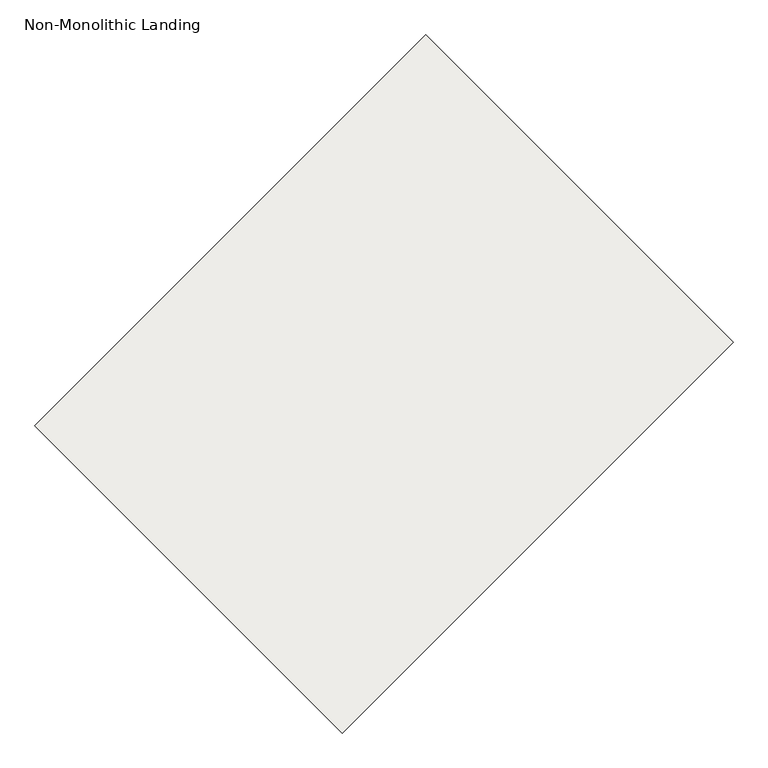
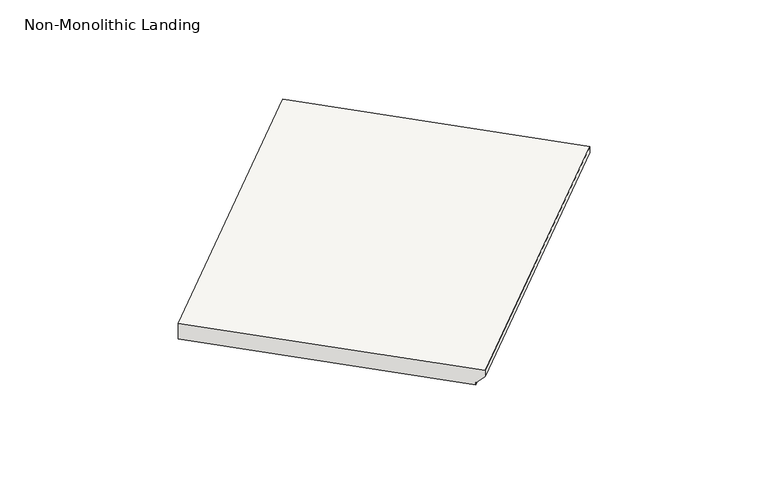
"""IFC4 building model written with IfcOpenShell, lengths in millimetres: slab geometry, Non-Monolithic Landing."""

from ifc_helpers import new_model, si_unit, frame, origin, place, context, project, spatial, polyline, outline, extrude, source, transform, mapped, element, save


def non_monolithic_landing_d434ce01(model_context):
    return source(origin(), model_context, "Body", "SweptSolid", [
        extrude(outline(polyline([(0.0, -838.2), (0.0, 0.0), (50.8, 0.0), (50.8, -812.8), (44.45, -812.8), (19.05, -838.2), (0.0, -838.2)])), frame((54022.1357118, -3599.6673453, 2870.2), z_axis=(0.7071067811865469, 0.7071067811865482, 0.0), x_axis=(0.0, 0.0, -1.0)), (0.0, 0.0, 1.0), 1066.8),
    ])


if __name__ == "__main__":
    model = new_model("IFC4")
    model_context = context("Model", 3, world=origin())
    ifc_project = project(units=[si_unit("LENGTHUNIT", "METRE", prefix="MILLI")], contexts=[model_context])
    site = spatial("IfcSite", under=ifc_project)
    building = spatial("IfcBuilding", under=site)
    placement = place(None, origin())
    non_monolithic_landing_shape = non_monolithic_landing_d434ce01(model_context)
    element("IfcSlab", 1, ObjectType="Non-Monolithic Landing", at=placement, inside=building, context=model_context, shape_type="MappedRepresentation", body=[
        mapped(non_monolithic_landing_shape, transform((0.0, 0.0, 0.0), x_axis=(1.0, 0.0, 0.0), y_axis=(0.0, 1.0, 0.0), z_axis=(0.0, 0.0, 1.0))),
    ])
    save(model, "model.ifc")

# Revit data of these elements
# Element 1 (IfcSlab, "Non-Monolithic Landing")
#   Materials on its faces: "Oak Flooring"
# Materials
#   "Oak Flooring": class "Wood", colour RGB 216 169 114, transparency 0, Description = "Quercus Rubra", Cost = 0
